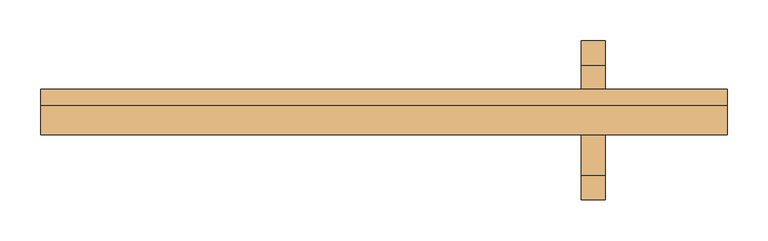
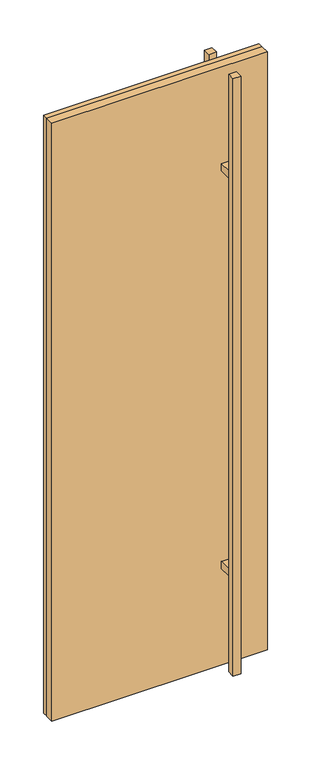
"""IFC4 building model written with IfcOpenShell, lengths in millimetres: door geometry, Anta Singola (1) : Anta Singola (1)."""

import ifcopenshell
import ifcopenshell.guid

model = None  # the IFC model being written
_history = None  # IfcOwnerHistory: only IFC2X3 demands one
_inside = {}  # id of a spatial element -> (the spatial element, [elements in it])
_under = {}  # id of a project, library or spatial element -> (it, [spatial elements below it])
_declared = {}  # id of a project -> (the project, [libraries it declares])
_typed = {}  # id of a type object -> (the type object, [elements of that type])
_made_of = {}  # id of a material, layer set ... -> (it, [elements and type objects made of it])


def new_model(schema):
    """Start an empty IFC model of exactly this schema.

    Asked for "IFC4X3", IfcOpenShell would pick the latest addendum, in which some entities
    have other attributes; the version numbers below select the first issue.
    IFC2X3 requires an IfcOwnerHistory on every rooted entity: one is made here for all.
    """
    global model, _history
    if schema == "IFC4X3":
        model = ifcopenshell.file(schema_version=(4, 3, 0, 0))
    else:
        model = ifcopenshell.file(schema=schema)
    _inside.clear()
    _under.clear()
    _declared.clear()
    _typed.clear()
    _made_of.clear()
    _history = None
    if model.schema == "IFC2X3":
        org = make("IfcOrganization", Name="unknown")
        user = make(
            "IfcPersonAndOrganization",
            ThePerson=make("IfcPerson", FamilyName="unknown"),
            TheOrganization=org,
        )
        app = make(
            "IfcApplication",
            ApplicationDeveloper=org,
            Version="unknown",
            ApplicationFullName="unknown",
            ApplicationIdentifier="unknown",
        )
        _history = make(
            "IfcOwnerHistory",
            OwningUser=user,
            OwningApplication=app,
            ChangeAction="ADDED",
            CreationDate=0,
        )
    return model


def make(cls, **values):
    """One entity of the class cls with the attributes given. An attribute that is None is left unset."""
    return model.create_entity(
        cls, **{name: value for name, value in values.items() if value is not None}
    )


def rooted(cls, **values):
    """An entity with a GlobalId (a new one), such as an element, a storey or a relation."""
    return make(cls, GlobalId=ifcopenshell.guid.new(), OwnerHistory=_history, **values)


def si_unit(unit_type, name, prefix=None):
    """IfcSIUnit, for example si_unit("LENGTHUNIT", "METRE", prefix="MILLI")."""
    return make("IfcSIUnit", UnitType=unit_type, Prefix=prefix, Name=name)


def assignment(units):
    """IfcUnitAssignment: the units of a project."""
    return None if units is None else make("IfcUnitAssignment", Units=units)


def point(xyz):
    """IfcCartesianPoint."""
    return None if xyz is None else make("IfcCartesianPoint", Coordinates=xyz)


def direction(xyz):
    """IfcDirection."""
    return None if xyz is None else make("IfcDirection", DirectionRatios=xyz)


def frame(location, z_axis=None, x_axis=None):
    """IfcAxis2Placement3D, a coordinate frame: its origin and axes. An axis left out is left unset."""
    return make(
        "IfcAxis2Placement3D",
        Location=point(location),
        Axis=direction(z_axis),
        RefDirection=direction(x_axis),
    )


def origin():
    """The frame at (0, 0, 0) with its axes left unset."""
    return frame((0.0, 0.0, 0.0))


def origin_with_axes():
    """The frame at (0, 0, 0) with the z axis (0, 0, 1) and the x axis (1, 0, 0) written out."""
    return frame((0.0, 0.0, 0.0), z_axis=(0.0, 0.0, 1.0), x_axis=(1.0, 0.0, 0.0))


def place(relative_to, where):
    """IfcLocalPlacement: puts the frame where relative to a parent placement (None: the world)."""
    return make(
        "IfcLocalPlacement", PlacementRelTo=relative_to, RelativePlacement=where
    )


def context(
    kind, dimensions, precision=None, world=None, true_north=None, identifier=None
):
    """IfcGeometricRepresentationContext, for example the 3D "Model" context."""
    return make(
        "IfcGeometricRepresentationContext",
        ContextIdentifier=identifier,
        ContextType=kind,
        CoordinateSpaceDimension=dimensions,
        Precision=precision,
        WorldCoordinateSystem=world,
        TrueNorth=true_north,
    )


def project(units=None, contexts=None):
    """IfcProject with its units and contexts."""
    return rooted(
        "IfcProject",
        Name="project",
        RepresentationContexts=contexts,
        UnitsInContext=assignment(units),
    )


def spatial(cls, under=None, at=None, **own):
    """A site, building, storey or space (cls), placed at a placement, below another one or the project."""
    s = rooted(cls, ObjectPlacement=at, **own)
    if under is not None:
        _under.setdefault(under.id(), (under, []))[1].append(s)
    return s


def polyline(points):
    """IfcPolyline through the points."""
    return make("IfcPolyline", Points=[point(p) for p in points])


def outline(outer, holes=None, kind="AREA"):
    """IfcArbitraryClosedProfileDef: a profile drawn as a closed curve; with holes, ...WithVoids."""
    if holes is None:
        return make("IfcArbitraryClosedProfileDef", ProfileType=kind, OuterCurve=outer)
    return make(
        "IfcArbitraryProfileDefWithVoids",
        ProfileType=kind,
        OuterCurve=outer,
        InnerCurves=holes,
    )


def extrude(swept, where, along, depth):
    """IfcExtrudedAreaSolid: the profile swept, set in the frame where, extruded along a direction by depth."""
    return make(
        "IfcExtrudedAreaSolid",
        SweptArea=swept,
        Position=where,
        ExtrudedDirection=direction(along),
        Depth=depth,
    )


def shape(context_of_items, identifier, shape_type, items):
    """IfcShapeRepresentation: the items that make up one representation, for example the "Body"."""
    return make(
        "IfcShapeRepresentation",
        ContextOfItems=context_of_items,
        RepresentationIdentifier=identifier,
        RepresentationType=shape_type,
        Items=items,
    )


def source(mapping_origin, context_of_items, identifier, shape_type, items):
    """IfcRepresentationMap: a shape defined once, which mapped items show again and again."""
    return make(
        "IfcRepresentationMap",
        MappingOrigin=mapping_origin,
        MappedRepresentation=shape(context_of_items, identifier, shape_type, items),
    )


def transform(
    local_origin,
    x_axis=None,
    y_axis=None,
    z_axis=None,
    scale=None,
    scale2=None,
    scale3=None,
    uniform=True,
):
    """IfcCartesianTransformationOperator3D, or its non-uniform kind. x_axis, y_axis, z_axis: its Axis1, 2, 3."""
    if uniform:
        return make(
            "IfcCartesianTransformationOperator3D",
            Axis1=direction(x_axis),
            Axis2=direction(y_axis),
            LocalOrigin=point(local_origin),
            Scale=scale,
            Axis3=direction(z_axis),
        )
    return make(
        "IfcCartesianTransformationOperator3DnonUniform",
        Axis1=direction(x_axis),
        Axis2=direction(y_axis),
        LocalOrigin=point(local_origin),
        Scale=scale,
        Axis3=direction(z_axis),
        Scale2=scale2,
        Scale3=scale3,
    )


def mapped(mapping_source, mapping_target):
    """IfcMappedItem: shows the shape of a source again, moved by a transform."""
    return make(
        "IfcMappedItem", MappingSource=mapping_source, MappingTarget=mapping_target
    )


def made_of(thing, what):
    """Note that an element or type object is made of a material, layer set ...; save() writes the relation."""
    if what is not None:
        _made_of.setdefault(what.id(), (what, []))[1].append(thing)
    return thing


def element(
    cls,
    number,
    at=None,
    inside=None,
    cuts=None,
    type_object=None,
    material=None,
    context=None,
    identifier="Body",
    shape_type=None,
    held_by="IfcProductDefinitionShape",
    body=None,
    shapes=None,
    **own,
):
    """One element of the class cls, such as IfcWall. Its Tag is "e" and its number.

    at: its placement. inside: the storey or other place that contains it. cuts: it is an
    opening in that element (IfcRelVoidsElement). A single representation is given by context,
    identifier, shape_type and body (its items); several are given by shapes. held_by: the class
    of the entity that holds the representations. save() writes the other relations.
    """
    e = rooted(cls, Tag="e%d" % number, ObjectPlacement=at, **own)
    if body is not None:
        shapes = [shape(context, identifier, shape_type, body)]
    if shapes is not None:
        e.Representation = make(held_by, Representations=shapes)
    if inside is not None:
        _inside.setdefault(inside.id(), (inside, []))[1].append(e)
    if cuts is not None:
        rooted(
            "IfcRelVoidsElement", RelatingBuildingElement=cuts, RelatedOpeningElement=e
        )
    if type_object is not None:
        _typed.setdefault(type_object.id(), (type_object, []))[1].append(e)
    return made_of(e, material)


def aggregate(whole, parts):
    """IfcRelAggregates: a whole, such as a stair, and the parts it consists of."""
    return rooted("IfcRelAggregates", RelatingObject=whole, RelatedObjects=parts)


def save(model, path):
    """Write the relations noted so far, then the file.

    IfcRelAggregates (storeys below a building ...), IfcRelContainedInSpatialStructure (elements
    in a storey), IfcRelDefinesByType, IfcRelAssociatesMaterial and IfcRelDeclares: one each for
    every whole, place, type object, material and project.
    """
    for whole, parts in _under.values():
        aggregate(whole, parts)
    for where, things in _inside.values():
        rooted(
            "IfcRelContainedInSpatialStructure",
            RelatedElements=things,
            RelatingStructure=where,
        )
    for kind, things in _typed.values():
        rooted("IfcRelDefinesByType", RelatedObjects=things, RelatingType=kind)
    for what, things in _made_of.values():
        rooted("IfcRelAssociatesMaterial", RelatedObjects=things, RelatingMaterial=what)
    for by, libraries in _declared.values():
        rooted("IfcRelDeclares", RelatingContext=by, RelatedDefinitions=libraries)
    model.write(path)


def door_ad57e7cc(model_context):
    return source(origin(), model_context, "Body", "SweptSolid", [
        extrude(outline(polyline([(422.5, 18.0), (422.5, -18.0), (-422.5, -18.0), (-422.5, 18.0), (422.5, 18.0)])), frame((0.0, 0.0, -3.1739529), z_axis=(0.0, 0.0, 1.0), x_axis=(1.0, 0.0, 0.0)), (0.0, 0.0, 1.0), 2478.1739529),
        extrude(outline(polyline([(242.5, 68.0), (242.5, 98.0), (272.5, 98.0), (272.5, 68.0), (242.5, 68.0)])), origin_with_axes(), (0.0, 0.0, 1.0), 2475.0),
        extrude(outline(polyline([(242.5, -98.0), (242.5, -68.0), (272.5, -68.0), (272.5, -98.0), (242.5, -98.0)])), origin_with_axes(), (0.0, 0.0, 1.0), 2475.0),
        extrude(outline(polyline([(2474.5625024, -422.0625024), (-2.7364552, -422.0625024), (-2.7364552, 422.0625024), (2474.5625024, 422.0625024), (2474.5625024, -422.0625024)]), holes=[polyline([(2429.5625024, 377.0625024), (42.2635448, 377.0625024), (42.2635448, -377.0625024), (2429.5625024, -377.0625024), (2429.5625024, 377.0625024)])]), frame((0.0, 18.0, 0.0), z_axis=(0.0, 1.0, 0.0), x_axis=(0.0, 0.0, 1.0)), (0.0, 0.0, 1.0), 20.0),
        extrude(outline(polyline([(272.5, -68.0), (242.5, -68.0), (242.5, -18.0), (272.5, -18.0), (272.5, -68.0)])), frame((0.0, 0.0, 396.8260471), z_axis=(0.0, 0.0, 1.0), x_axis=(1.0, 0.0, 0.0)), (0.0, 0.0, 1.0), 30.0),
        extrude(outline(polyline([(272.5, -68.0), (242.5, -68.0), (242.5, -18.0), (272.5, -18.0), (272.5, -68.0)])), frame((0.0, 0.0, 2045.0), z_axis=(0.0, 0.0, 1.0), x_axis=(1.0, 0.0, 0.0)), (0.0, 0.0, 1.0), 30.0),
        extrude(outline(polyline([(272.5, 18.0), (242.5, 18.0), (242.5, 68.0), (272.5, 68.0), (272.5, 18.0)])), frame((0.0, 0.0, 396.8260471), z_axis=(0.0, 0.0, 1.0), x_axis=(1.0, 0.0, 0.0)), (0.0, 0.0, 1.0), 30.0),
        extrude(outline(polyline([(272.5, 18.0), (242.5, 18.0), (242.5, 68.0), (272.5, 68.0), (272.5, 18.0)])), frame((0.0, 0.0, 2045.0), z_axis=(0.0, 0.0, 1.0), x_axis=(1.0, 0.0, 0.0)), (0.0, 0.0, 1.0), 30.0),
    ])


if __name__ == "__main__":
    model = new_model("IFC4")
    model_context = context("Model", 3, world=origin())
    ifc_project = project(units=[si_unit("LENGTHUNIT", "METRE", prefix="MILLI")], contexts=[model_context])
    site = spatial("IfcSite", under=ifc_project)
    building = spatial("IfcBuilding", under=site)
    placement = place(None, origin())
    door_shape = door_ad57e7cc(model_context)
    element("IfcDoor", 1, ObjectType="Anta Singola (1) : Anta Singola (1)", at=placement, inside=building, context=model_context, shape_type="MappedRepresentation", body=[
        mapped(door_shape, transform((0.0, 0.0, 0.0), x_axis=(1.0, 0.0, 0.0), y_axis=(0.0, 1.0, 0.0), z_axis=(0.0, 0.0, 1.0))),
    ])
    save(model, "model.ifc")

# Revit data of these elements
# Type "Anta Singola (1) : Anta Singola (1)"
#   Type Mark = "13"
#   Operation = ""
#   Construction Type = "Scorrimenti"
#   Construction Type Id = "opn-d42"
#   Analytic Construction = "Telaio in metallo con vetro singolo trasparente"
#   Sp = 0.036 m
#   Heat Transfer Coefficient (U) = 6.5580 W/(m²·K)
#   L cornice = 0.045 m
#   Quadro = Default - Vetro
#   Maniglia = none
#   Visual Light Transmittance = 0
#   Solar Heat Gain Coefficient = 0
#   Manufacturer = ""
#   Function = (empty or 0)
# Element 1 (IfcDoor, "Anta Singola (1) : Anta Singola (1)")
#   Materials on its faces: "Maniglia", "Default - Vetro"
# Materials
#   "Default - Vetro": class "Vetro", colour RGB 208 208 208, transparency 0.7, Cost = 0
#   "Maniglia": class "Varie", colour RGB 219 219 219, transparency 0
